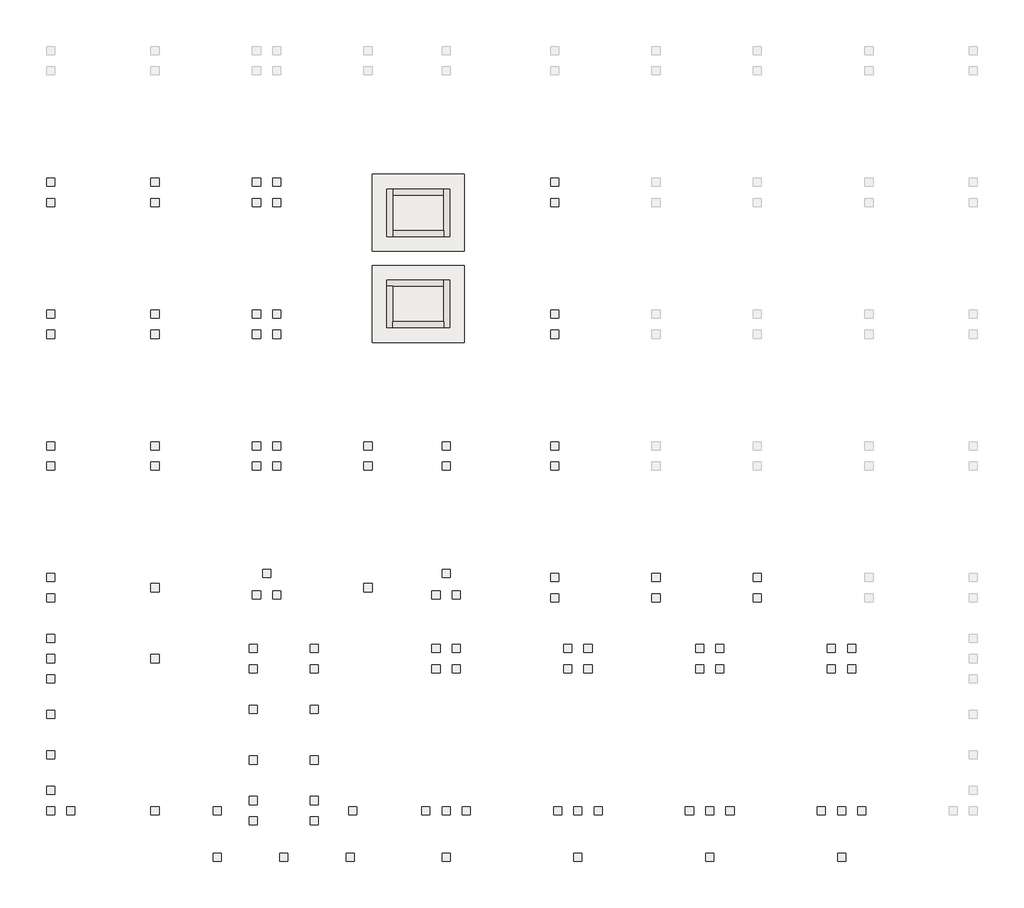
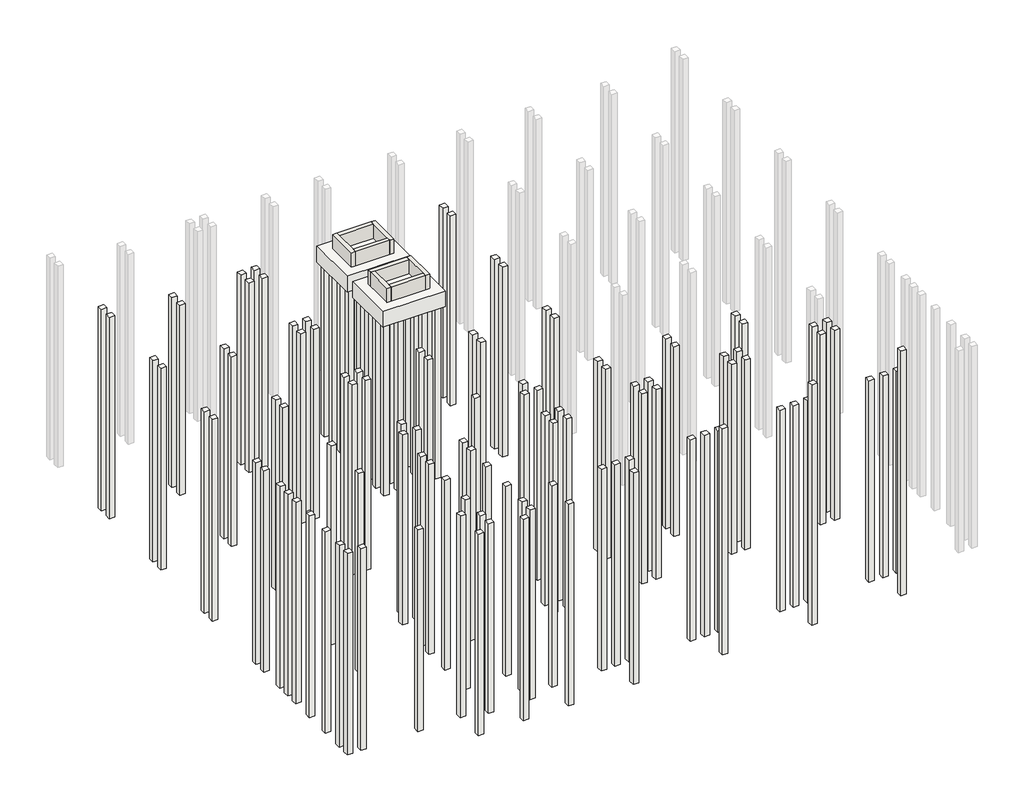
# Not in any storey, part 1 of 2: 143 footings, 8 walls.
# Revit data of these elements (continued)
# Element 100 (IfcFooting, "NLRS_17_SFO_TLB_funderingspaal geheid beton prefab-AV-MMBPC_gen_rsf : heipaal beton prefab_gen__bxh 400x400")
#   IfcGUID = "3loy75XKz2Rw4dS8JWiaqH"
#   Slanted Angle = 0.00°
#   NLRS_S_draagvermogen_trek = 0.00 kN
#   NLRS_S_draagvermogen_druk = 0.00 kN
#   Angle = 0.00°
#   IsExternal = yes
#   LoadBearing = yes
#   Slanted = 0
#   Phase Created = NLRS_nieuw
#   Materials on its faces: "NLRS_f2_beton prefab_gen_rsf"
# Element 101 (IfcFooting, "NLRS_17_SFO_TLB_funderingspaal geheid beton prefab-AV-MMBPC_gen_rsf : heipaal beton prefab_gen__bxh 400x400")
#   IfcGUID = "3loy75XKz2Rw4dS8JWiaqU"
#   Slanted Angle = 0.00°
#   NLRS_S_draagvermogen_trek = 0.00 kN
#   NLRS_S_draagvermogen_druk = 0.00 kN
#   Angle = 0.00°
#   IsExternal = yes
#   LoadBearing = yes
#   Slanted = 0
#   Phase Created = NLRS_nieuw
#   Materials on its faces: "NLRS_f2_beton prefab_gen_rsf"
# Element 102 (IfcFooting, "NLRS_17_SFO_TLB_funderingspaal geheid beton prefab-AV-MMBPC_gen_rsf : heipaal beton prefab_gen__bxh 400x400")
#   IfcGUID = "3loy75XKz2Rw4dS8JWiaqS"
#   Slanted Angle = 0.00°
#   NLRS_S_draagvermogen_trek = 0.00 kN
#   NLRS_S_draagvermogen_druk = 0.00 kN
#   Angle = 0.00°
#   IsExternal = yes
#   LoadBearing = yes
#   Slanted = 0
#   Phase Created = NLRS_nieuw
#   Materials on its faces: "NLRS_f2_beton prefab_gen_rsf"
# Element 103 (IfcFooting, "NLRS_17_SFO_TLB_funderingspaal geheid beton prefab-AV-MMBPC_gen_rsf : heipaal beton prefab_gen__bxh 400x400")
#   IfcGUID = "3loy75XKz2Rw4dS8JWiaq9"
#   Slanted Angle = 0.00°
#   NLRS_S_draagvermogen_trek = 0.00 kN
#   NLRS_S_draagvermogen_druk = 0.00 kN
#   Angle = 0.00°
#   IsExternal = yes
#   LoadBearing = yes
#   Slanted = 0
#   Phase Created = NLRS_nieuw
#   Materials on its faces: "NLRS_f2_beton prefab_gen_rsf"
# Element 104 (IfcFooting, "NLRS_17_SFO_TLB_funderingspaal geheid beton prefab-AV-MMBPC_gen_rsf : heipaal beton prefab_gen__bxh 400x400")
#   IfcGUID = "3loy75XKz2Rw4dS8JWiaqF"
#   Slanted Angle = 0.00°
#   NLRS_S_draagvermogen_trek = 0.00 kN
#   NLRS_S_draagvermogen_druk = 0.00 kN
#   Angle = 0.00°
#   IsExternal = yes
#   LoadBearing = yes
#   Slanted = 0
#   Phase Created = NLRS_nieuw
#   Materials on its faces: "NLRS_f2_beton prefab_gen_rsf"
# Element 105 (IfcFooting, "NLRS_17_SFO_TLB_funderingspaal geheid beton prefab-AV-MMBPC_gen_rsf : heipaal beton prefab_gen__bxh 400x400")
#   IfcGUID = "3loy75XKz2Rw4dS8JWia7f"
#   Slanted Angle = 0.00°
#   NLRS_S_draagvermogen_trek = 0.00 kN
#   NLRS_S_draagvermogen_druk = 0.00 kN
#   Angle = 0.00°
#   IsExternal = yes
#   LoadBearing = yes
#   Slanted = 0
#   Phase Created = NLRS_nieuw
#   Materials on its faces: "NLRS_f2_beton prefab_gen_rsf"
# Element 106 (IfcFooting, "NLRS_17_SFO_TLB_funderingspaal geheid beton prefab-AV-MMBPC_gen_rsf : heipaal beton prefab_gen__bxh 400x400")
#   IfcGUID = "3loy75XKz2Rw4dS8JWia6M"
#   Slanted Angle = 0.00°
#   NLRS_S_draagvermogen_trek = 0.00 kN
#   NLRS_S_draagvermogen_druk = 0.00 kN
#   Angle = 0.00°
#   IsExternal = yes
#   LoadBearing = yes
#   Slanted = 0
#   Phase Created = NLRS_nieuw
#   Materials on its faces: "NLRS_f2_beton prefab_gen_rsf"
# Element 107 (IfcFooting, "NLRS_17_SFO_TLB_funderingspaal geheid beton prefab-AV-MMBPC_gen_rsf : heipaal beton prefab_gen__bxh 400x400")
#   IfcGUID = "3loy75XKz2Rw4dS8JWiaPz"
#   Slanted Angle = 0.00°
#   NLRS_S_draagvermogen_trek = 0.00 kN
#   NLRS_S_draagvermogen_druk = 0.00 kN
#   Angle = 0.00°
#   IsExternal = yes
#   LoadBearing = yes
#   Slanted = 0
#   Phase Created = NLRS_nieuw
#   Materials on its faces: "NLRS_f2_beton prefab_gen_rsf"
# Element 108 (IfcFooting, "NLRS_17_SFO_TLB_funderingspaal geheid beton prefab-AV-MMBPC_gen_rsf : heipaal beton prefab_gen__bxh 400x400")
#   IfcGUID = "3yoae3mAzBRekDMiYpsxUC"
#   Slanted Angle = 0.00°
#   NLRS_S_draagvermogen_trek = 0.00 kN
#   NLRS_S_draagvermogen_druk = 0.00 kN
#   Angle = 0.00°
#   IsExternal = yes
#   LoadBearing = yes
#   Slanted = 0
#   Phase Created = NLRS_nieuw
#   Materials on its faces: "NLRS_f2_beton prefab_gen_rsf"
# Element 109 (IfcFooting, "NLRS_17_SFO_TLB_funderingspaal geheid beton prefab-AV-MMBPC_gen_rsf : heipaal beton prefab_gen__bxh 400x400")
#   IfcGUID = "3yoae3mAzBRekDMiYpsxUN"
#   Slanted Angle = 0.00°
#   NLRS_S_draagvermogen_trek = 0.00 kN
#   NLRS_S_draagvermogen_druk = 0.00 kN
#   Angle = 0.00°
#   IsExternal = yes
#   LoadBearing = yes
#   Slanted = 0
#   Phase Created = NLRS_nieuw
#   Materials on its faces: "NLRS_f2_beton prefab_gen_rsf"
# Element 110 (IfcFooting, "NLRS_17_SFO_TLB_funderingspaal geheid beton prefab-AV-MMBPC_gen_rsf : heipaal beton prefab_gen__bxh 400x400")
#   IfcGUID = "3yoae3mAzBRekDMiYpsxUU"
#   Slanted Angle = 0.00°
#   NLRS_S_draagvermogen_trek = 0.00 kN
#   NLRS_S_draagvermogen_druk = 0.00 kN
#   Angle = 0.00°
#   IsExternal = yes
#   LoadBearing = yes
#   Slanted = 0
#   Phase Created = NLRS_nieuw
#   Materials on its faces: "NLRS_f2_beton prefab_gen_rsf"
# Element 111 (IfcFooting, "NLRS_17_SFO_TLB_funderingspaal geheid beton prefab-AV-MMBPC_gen_rsf : heipaal beton prefab_gen__bxh 400x400")
#   IfcGUID = "3yoae3mAzBRekDMiYpsxVf"
#   Slanted Angle = 0.00°
#   NLRS_S_draagvermogen_trek = 0.00 kN
#   NLRS_S_draagvermogen_druk = 0.00 kN
#   Angle = 0.00°
#   IsExternal = yes
#   LoadBearing = yes
#   Slanted = 0
#   Phase Created = NLRS_nieuw
#   Materials on its faces: "NLRS_f2_beton prefab_gen_rsf"
# Element 112 (IfcFooting, "NLRS_17_SFO_TLB_funderingspaal geheid beton prefab-AV-MMBPC_gen_rsf : heipaal beton prefab_gen__bxh 400x400")
#   IfcGUID = "22y6L5gAz9AR8RjJaZzOrs"
#   Slanted Angle = 0.00°
#   NLRS_S_draagvermogen_trek = 0.00 kN
#   NLRS_S_draagvermogen_druk = 0.00 kN
#   Angle = 0.00°
#   IsExternal = yes
#   LoadBearing = yes
#   Slanted = 0
#   Phase Created = NLRS_nieuw
#   Materials on its faces: "NLRS_f2_beton prefab_gen_rsf"
# Element 113 (IfcFooting, "NLRS_17_SFO_TLB_funderingspaal geheid beton prefab-AV-MMBPC_gen_rsf : heipaal beton prefab_gen__bxh 400x400")
#   IfcGUID = "22y6L5gAz9AR8RjJaZzOqH"
#   Slanted Angle = 0.00°
#   NLRS_S_draagvermogen_trek = 0.00 kN
#   NLRS_S_draagvermogen_druk = 0.00 kN
#   Angle = 0.00°
#   IsExternal = yes
#   LoadBearing = yes
#   Slanted = 0
#   Phase Created = NLRS_nieuw
#   Materials on its faces: "NLRS_f2_beton prefab_gen_rsf"
# Element 114 (IfcFooting, "NLRS_17_SFO_TLB_funderingspaal geheid beton prefab-AV-MMBPC_gen_rsf : heipaal beton prefab_gen__bxh 400x400")
#   IfcGUID = "22y6L5gAz9AR8RjJaZzOo$"
#   Slanted Angle = 0.00°
#   NLRS_S_draagvermogen_trek = 0.00 kN
#   NLRS_S_draagvermogen_druk = 0.00 kN
#   Angle = 0.00°
#   IsExternal = yes
#   LoadBearing = yes
#   Slanted = 0
#   Phase Created = NLRS_nieuw
#   Materials on its faces: "NLRS_f2_beton prefab_gen_rsf"
# Element 115 (IfcFooting, "NLRS_17_SFO_TLB_funderingspaal geheid beton prefab-AV-MMBPC_gen_rsf : heipaal beton prefab_gen__bxh 400x400")
#   IfcGUID = "22y6L5gAz9AR8RjJaZzOn6"
#   Slanted Angle = 0.00°
#   NLRS_S_draagvermogen_trek = 0.00 kN
#   NLRS_S_draagvermogen_druk = 0.00 kN
#   Angle = 0.00°
#   IsExternal = yes
#   LoadBearing = yes
#   Slanted = 0
#   Phase Created = NLRS_nieuw
#   Materials on its faces: "NLRS_f2_beton prefab_gen_rsf"
# Element 116 (IfcFooting, "NLRS_17_SFO_TLB_funderingspaal geheid beton prefab-AV-MMBPC_gen_rsf : heipaal beton prefab_gen__bxh 400x400")
#   IfcGUID = "22y6L5gAz9AR8RjJaZzOmJ"
#   Slanted Angle = 0.00°
#   NLRS_S_draagvermogen_trek = 0.00 kN
#   NLRS_S_draagvermogen_druk = 0.00 kN
#   Angle = 0.00°
#   IsExternal = yes
#   LoadBearing = yes
#   Slanted = 0
#   Phase Created = NLRS_nieuw
#   Materials on its faces: "NLRS_f2_beton prefab_gen_rsf"
# Element 117 (IfcFooting, "NLRS_17_SFO_TLB_funderingspaal geheid beton prefab-AV-MMBPC_gen_rsf : heipaal beton prefab_gen__bxh 400x400")
#   IfcGUID = "22y6L5gAz9AR8RjJaZzOmD"
#   Slanted Angle = 0.00°
#   NLRS_S_draagvermogen_trek = 0.00 kN
#   NLRS_S_draagvermogen_druk = 0.00 kN
#   Angle = 0.00°
#   IsExternal = yes
#   LoadBearing = yes
#   Slanted = 0
#   Phase Created = NLRS_nieuw
#   Materials on its faces: "NLRS_f2_beton prefab_gen_rsf"
# Element 118 (IfcFooting, "NLRS_17_SFO_TLB_funderingspaal geheid beton prefab-AV-MMBPC_gen_rsf : heipaal beton prefab_gen__bxh 400x400")
#   IfcGUID = "22y6L5gAz9AR8RjJaZzOmk"
#   Slanted Angle = 0.00°
#   NLRS_S_draagvermogen_trek = 0.00 kN
#   NLRS_S_draagvermogen_druk = 0.00 kN
#   Angle = 0.00°
#   IsExternal = yes
#   LoadBearing = yes
#   Slanted = 0
#   Phase Created = NLRS_nieuw
#   Materials on its faces: "NLRS_f2_beton prefab_gen_rsf"
# Element 119 (IfcFooting, "NLRS_17_SFO_TLB_funderingspaal geheid beton prefab-AV-MMBPC_gen_rsf : heipaal beton prefab_gen__bxh 400x400")
#   IfcGUID = "22y6L5gAz9AR8RjJaZzOme"
#   Slanted Angle = 0.00°
#   NLRS_S_draagvermogen_trek = 0.00 kN
#   NLRS_S_draagvermogen_druk = 0.00 kN
#   Angle = 0.00°
#   IsExternal = yes
#   LoadBearing = yes
#   Slanted = 0
#   Phase Created = NLRS_nieuw
#   Materials on its faces: "NLRS_f2_beton prefab_gen_rsf"
# Element 120 (IfcFooting, "NLRS_17_SFO_TLB_funderingspaal geheid beton prefab-AV-MMBPC_gen_rsf : heipaal beton prefab_gen__bxh 400x400")
#   IfcGUID = "22y6L5gAz9AR8RjJaZzO$2"
#   Slanted Angle = 0.00°
#   NLRS_S_draagvermogen_trek = 0.00 kN
#   NLRS_S_draagvermogen_druk = 0.00 kN
#   Angle = 0.00°
#   IsExternal = yes
#   LoadBearing = yes
#   Slanted = 0
#   Phase Created = NLRS_nieuw
#   Materials on its faces: "NLRS_f2_beton prefab_gen_rsf"
# Element 121 (IfcFooting, "NLRS_17_SFO_TLB_funderingspaal geheid beton prefab-AV-MMBPC_gen_rsf : heipaal beton prefab_gen__bxh 400x400")
#   IfcGUID = "22y6L5gAz9AR8RjJaZzO$y"
#   Slanted Angle = 0.00°
#   NLRS_S_draagvermogen_trek = 0.00 kN
#   NLRS_S_draagvermogen_druk = 0.00 kN
#   Angle = 0.00°
#   IsExternal = yes
#   LoadBearing = yes
#   Slanted = 0
#   Phase Created = NLRS_nieuw
#   Materials on its faces: "NLRS_f2_beton prefab_gen_rsf"
# Element 122 (IfcFooting, "NLRS_17_SFO_TLB_funderingspaal geheid beton prefab-AV-MMBPC_gen_rsf : heipaal beton prefab_gen__bxh 400x400")
#   IfcGUID = "22y6L5gAz9AR8RjJaZzO$_"
#   Slanted Angle = 0.00°
#   NLRS_S_draagvermogen_trek = 0.00 kN
#   NLRS_S_draagvermogen_druk = 0.00 kN
#   Angle = 0.00°
#   IsExternal = yes
#   LoadBearing = yes
#   Slanted = 0
#   Phase Created = NLRS_nieuw
#   Materials on its faces: "NLRS_f2_beton prefab_gen_rsf"
# Element 123 (IfcFooting, "NLRS_17_SFO_TLB_funderingspaal geheid beton prefab-AV-MMBPC_gen_rsf : heipaal beton prefab_gen__bxh 400x400")
#   IfcGUID = "22y6L5gAz9AR8RjJaZzO$u"
#   Slanted Angle = 0.00°
#   NLRS_S_draagvermogen_trek = 0.00 kN
#   NLRS_S_draagvermogen_druk = 0.00 kN
#   Angle = 0.00°
#   IsExternal = yes
#   LoadBearing = yes
#   Slanted = 0
#   Phase Created = NLRS_nieuw
#   Materials on its faces: "NLRS_f2_beton prefab_gen_rsf"
# Element 124 (IfcFooting, "NLRS_17_SFO_TLB_funderingspaal geheid beton prefab-AV-MMBPC_gen_rsf : heipaal beton prefab_gen__bxh 400x400")
#   IfcGUID = "22y6L5gAz9AR8RjJaZzO$w"
#   Slanted Angle = 0.00°
#   NLRS_S_draagvermogen_trek = 0.00 kN
#   NLRS_S_draagvermogen_druk = 0.00 kN
#   Angle = 0.00°
#   IsExternal = yes
#   LoadBearing = yes
#   Slanted = 0
#   Phase Created = NLRS_nieuw
#   Materials on its faces: "NLRS_f2_beton prefab_gen_rsf"
# Element 125 (IfcFooting, "NLRS_17_SFO_TLB_funderingspaal geheid beton prefab-AV-MMBPC_gen_rsf : heipaal beton prefab_gen__bxh 400x400")
#   IfcGUID = "22y6L5gAz9AR8RjJaZzO$q"
#   Slanted Angle = 0.00°
#   NLRS_S_draagvermogen_trek = 0.00 kN
#   NLRS_S_draagvermogen_druk = 0.00 kN
#   Angle = 0.00°
#   IsExternal = yes
#   LoadBearing = yes
#   Slanted = 0
#   Phase Created = NLRS_nieuw
#   Materials on its faces: "NLRS_f2_beton prefab_gen_rsf"
# Element 126 (IfcFooting, "NLRS_17_SFO_TLB_funderingspaal geheid beton prefab-AV-MMBPC_gen_rsf : heipaal beton prefab_gen__bxh 400x400")
#   IfcGUID = "22y6L5gAz9AR8RjJaZzO$s"
#   Slanted Angle = 0.00°
#   NLRS_S_draagvermogen_trek = 0.00 kN
#   NLRS_S_draagvermogen_druk = 0.00 kN
#   Angle = 0.00°
#   IsExternal = yes
#   LoadBearing = yes
#   Slanted = 0
#   Phase Created = NLRS_nieuw
#   Materials on its faces: "NLRS_f2_beton prefab_gen_rsf"
# Element 127 (IfcFooting, "NLRS_17_SFO_TLB_funderingspaal geheid beton prefab-AV-MMBPC_gen_rsf : heipaal beton prefab_gen__bxh 400x400")
#   IfcGUID = "22y6L5gAz9AR8RjJaZzO$m"
#   Slanted Angle = 0.00°
#   NLRS_S_draagvermogen_trek = 0.00 kN
#   NLRS_S_draagvermogen_druk = 0.00 kN
#   Angle = 0.00°
#   IsExternal = yes
#   LoadBearing = yes
#   Slanted = 0
#   Phase Created = NLRS_nieuw
#   Materials on its faces: "NLRS_f2_beton prefab_gen_rsf"
# Element 128 (IfcFooting, "NLRS_17_SFO_TLB_funderingspaal geheid beton prefab-AV-MMBPC_gen_rsf : heipaal beton prefab_gen__bxh 400x400")
#   IfcGUID = "22y6L5gAz9AR8RjJaZzOuC"
#   Slanted Angle = 0.00°
#   NLRS_S_draagvermogen_trek = 0.00 kN
#   NLRS_S_draagvermogen_druk = 0.00 kN
#   Angle = 0.00°
#   IsExternal = yes
#   LoadBearing = yes
#   Slanted = 0
#   Phase Created = NLRS_nieuw
#   Materials on its faces: "NLRS_f2_beton prefab_gen_rsf"
# Element 129 (IfcFooting, "NLRS_17_SFO_TLB_funderingspaal geheid beton prefab-AV-MMBPC_gen_rsf : heipaal beton prefab_gen__bxh 400x400")
#   IfcGUID = "22y6L5gAz9AR8RjJaZzOuE"
#   Slanted Angle = 0.00°
#   NLRS_S_draagvermogen_trek = 0.00 kN
#   NLRS_S_draagvermogen_druk = 0.00 kN
#   Angle = 0.00°
#   IsExternal = yes
#   LoadBearing = yes
#   Slanted = 0
#   Phase Created = NLRS_nieuw
#   Materials on its faces: "NLRS_f2_beton prefab_gen_rsf"
# Element 130 (IfcFooting, "NLRS_17_SFO_TLB_funderingspaal geheid beton prefab-AV-MMBPC_gen_rsf : heipaal beton prefab_gen__bxh 400x400")
#   IfcGUID = "22y6L5gAz9AR8RjJaZzOu8"
#   Slanted Angle = 0.00°
#   NLRS_S_draagvermogen_trek = 0.00 kN
#   NLRS_S_draagvermogen_druk = 0.00 kN
#   Angle = 0.00°
#   IsExternal = yes
#   LoadBearing = yes
#   Slanted = 0
#   Phase Created = NLRS_nieuw
#   Materials on its faces: "NLRS_f2_beton prefab_gen_rsf"
# Element 131 (IfcFooting, "NLRS_17_SFO_TLB_funderingspaal geheid beton prefab-AV-MMBPC_gen_rsf : heipaal beton prefab_gen__bxh 400x400")
#   IfcGUID = "22y6L5gAz9AR8RjJaZzOuA"
#   Slanted Angle = 0.00°
#   NLRS_S_draagvermogen_trek = 0.00 kN
#   NLRS_S_draagvermogen_druk = 0.00 kN
#   Angle = 0.00°
#   IsExternal = yes
#   LoadBearing = yes
#   Slanted = 0
#   Phase Created = NLRS_nieuw
#   Materials on its faces: "NLRS_f2_beton prefab_gen_rsf"
# Element 132 (IfcFooting, "NLRS_17_SFO_TLB_funderingspaal geheid beton prefab-AV-MMBPC_gen_rsf : heipaal beton prefab_gen__bxh 400x400")
#   IfcGUID = "22y6L5gAz9AR8RjJaZzOu4"
#   Slanted Angle = 0.00°
#   NLRS_S_draagvermogen_trek = 0.00 kN
#   NLRS_S_draagvermogen_druk = 0.00 kN
#   Angle = 0.00°
#   IsExternal = yes
#   LoadBearing = yes
#   Slanted = 0
#   Phase Created = NLRS_nieuw
#   Materials on its faces: "NLRS_f2_beton prefab_gen_rsf"
# Element 133 (IfcFooting, "NLRS_17_SFO_TLB_funderingspaal geheid beton prefab-AV-MMBPC_gen_rsf : heipaal beton prefab_gen__bxh 400x400")
#   IfcGUID = "22y6L5gAz9AR8RjJaZzOu6"
#   Slanted Angle = 0.00°
#   NLRS_S_draagvermogen_trek = 0.00 kN
#   NLRS_S_draagvermogen_druk = 0.00 kN
#   Angle = 0.00°
#   IsExternal = yes
#   LoadBearing = yes
#   Slanted = 0
#   Phase Created = NLRS_nieuw
#   Materials on its faces: "NLRS_f2_beton prefab_gen_rsf"
# Element 134 (IfcFooting, "NLRS_17_SFO_TLB_funderingspaal geheid beton prefab-AV-MMBPC_gen_rsf : heipaal beton prefab_gen__bxh 400x400")
#   IfcGUID = "22y6L5gAz9AR8RjJaZzOu0"
#   Slanted Angle = 0.00°
#   NLRS_S_draagvermogen_trek = 0.00 kN
#   NLRS_S_draagvermogen_druk = 0.00 kN
#   Angle = 0.00°
#   IsExternal = yes
#   LoadBearing = yes
#   Slanted = 0
#   Phase Created = NLRS_nieuw
#   Materials on its faces: "NLRS_f2_beton prefab_gen_rsf"
# Element 135 (IfcFooting, "NLRS_17_SFO_TLB_funderingspaal geheid beton prefab-AV-MMBPC_gen_rsf : heipaal beton prefab_gen__bxh 400x400")
#   IfcGUID = "22y6L5gAz9AR8RjJaZzOu2"
#   Slanted Angle = 0.00°
#   NLRS_S_draagvermogen_trek = 0.00 kN
#   NLRS_S_draagvermogen_druk = 0.00 kN
#   Angle = 0.00°
#   IsExternal = yes
#   LoadBearing = yes
#   Slanted = 0
#   Phase Created = NLRS_nieuw
#   Materials on its faces: "NLRS_f2_beton prefab_gen_rsf"
# Element 136 (IfcFooting, "NLRS_17_SFO_TLB_funderingspaal geheid beton prefab-AV-MMBPC_gen_rsf : heipaal beton prefab_gen__bxh 400x400")
#   IfcGUID = "22y6L5gAz9AR8RjJaZzOuy"
#   Slanted Angle = 0.00°
#   NLRS_S_draagvermogen_trek = 0.00 kN
#   NLRS_S_draagvermogen_druk = 0.00 kN
#   Angle = 0.00°
#   IsExternal = yes
#   LoadBearing = yes
#   Slanted = 0
#   Phase Created = NLRS_nieuw
#   Materials on its faces: "NLRS_f2_beton prefab_gen_rsf"
# Element 137 (IfcFooting, "NLRS_17_SFO_TLB_funderingspaal geheid beton prefab-AV-MMBPC_gen_rsf : heipaal beton prefab_gen__bxh 400x400")
#   IfcGUID = "22y6L5gAz9AR8RjJaZzOu_"
#   Slanted Angle = 0.00°
#   NLRS_S_draagvermogen_trek = 0.00 kN
#   NLRS_S_draagvermogen_druk = 0.00 kN
#   Angle = 0.00°
#   IsExternal = yes
#   LoadBearing = yes
#   Slanted = 0
#   Phase Created = NLRS_nieuw
#   Materials on its faces: "NLRS_f2_beton prefab_gen_rsf"
# Element 138 (IfcFooting, "NLRS_17_SFO_TLB_funderingspaal geheid beton prefab-AV-MMBPC_gen_rsf : heipaal beton prefab_gen__bxh 400x400")
#   IfcGUID = "22y6L5gAz9AR8RjJaZzOuu"
#   Slanted Angle = 0.00°
#   NLRS_S_draagvermogen_trek = 0.00 kN
#   NLRS_S_draagvermogen_druk = 0.00 kN
#   Angle = 0.00°
#   IsExternal = yes
#   LoadBearing = yes
#   Slanted = 0
#   Phase Created = NLRS_nieuw
#   Materials on its faces: "NLRS_f2_beton prefab_gen_rsf"
# Element 139 (IfcFooting, "NLRS_17_SFO_TLB_funderingspaal geheid beton prefab-AV-MMBPC_gen_rsf : heipaal beton prefab_gen__bxh 400x400")
#   IfcGUID = "22y6L5gAz9AR8RjJaZzOuw"
#   Slanted Angle = 0.00°
#   NLRS_S_draagvermogen_trek = 0.00 kN
#   NLRS_S_draagvermogen_druk = 0.00 kN
#   Angle = 0.00°
#   IsExternal = yes
#   LoadBearing = yes
#   Slanted = 0
#   Phase Created = NLRS_nieuw
#   Materials on its faces: "NLRS_f2_beton prefab_gen_rsf"
# Element 140 (IfcFooting, "NLRS_17_SFO_TLB_funderingspaal geheid beton prefab-AV-MMBPC_gen_rsf : heipaal beton prefab_gen__bxh 400x400")
#   IfcGUID = "22y6L5gAz9AR8RjJaZzOuq"
#   Slanted Angle = 0.00°
#   NLRS_S_draagvermogen_trek = 0.00 kN
#   NLRS_S_draagvermogen_druk = 0.00 kN
#   Angle = 0.00°
#   IsExternal = yes
#   LoadBearing = yes
#   Slanted = 0
#   Phase Created = NLRS_nieuw
#   Materials on its faces: "NLRS_f2_beton prefab_gen_rsf"
# Element 141 (IfcFooting, "NLRS_17_SFO_TLB_funderingspaal geheid beton prefab-AV-MMBPC_gen_rsf : heipaal beton prefab_gen__bxh 400x400")
#   IfcGUID = "22y6L5gAz9AR8RjJaZzOus"
#   Slanted Angle = 0.00°
#   NLRS_S_draagvermogen_trek = 0.00 kN
#   NLRS_S_draagvermogen_druk = 0.00 kN
#   Angle = 0.00°
#   IsExternal = yes
#   LoadBearing = yes
#   Slanted = 0
#   Phase Created = NLRS_nieuw
#   Materials on its faces: "NLRS_f2_beton prefab_gen_rsf"
# Element 142 (IfcFooting, "NLRS_17_SFO_TLB_funderingspaal geheid beton prefab-AV-MMBPC_gen_rsf : heipaal beton prefab_gen__bxh 400x400")
#   IfcGUID = "22y6L5gAz9AR8RjJaZzOum"
#   Slanted Angle = 0.00°
#   NLRS_S_draagvermogen_trek = 0.00 kN
#   NLRS_S_draagvermogen_druk = 0.00 kN
#   Angle = 0.00°
#   IsExternal = yes
#   LoadBearing = yes
#   Slanted = 0
#   Phase Created = NLRS_nieuw
#   Materials on its faces: "NLRS_f2_beton prefab_gen_rsf"
# Element 143 (IfcFooting, "NLRS_17_SFO_TLB_funderingspaal geheid beton prefab-AV-MMBPC_gen_rsf : heipaal beton prefab_gen__bxh 400x400")
#   IfcGUID = "22y6L5gAz9AR8RjJaZzOuo"
#   Slanted Angle = 0.00°
#   NLRS_S_draagvermogen_trek = 0.00 kN
#   NLRS_S_draagvermogen_druk = 0.00 kN
#   Angle = 0.00°
#   IsExternal = yes
#   LoadBearing = yes
#   Slanted = 0
#   Phase Created = NLRS_nieuw
#   Materials on its faces: "NLRS_f2_beton prefab_gen_rsf"
# Element 144 (IfcWall, "NLRS_16_WA_beton ihw 300_gen_rsf")
#   IfcGUID = "22y6L5gAz9AR8RjJaZzOY4"
#   Comments = ""
#   Top Offset = 0 mm
#   Base Offset = 0 mm
#   wall height = 1100 mm
#   IsExternal = yes
#   LoadBearing = yes
#   Phase Created = NLRS_nieuw
#   Base Constraint = -02_bk ruwe vloer liftput
#   Top Constraint = -01_ok ruwe vloer
#   Materials on its faces: "NLRS_f2_beton ihwg_gen_rsf"
# Element 145 (IfcWall, "NLRS_16_WA_beton ihw 300_gen_rsf")
#   IfcGUID = "22y6L5gAz9AR8RjJaZzOY6"
#   Comments = ""
#   Top Offset = 0 mm
#   Base Offset = 0 mm
#   wall height = 1100 mm
#   IsExternal = yes
#   LoadBearing = yes
#   Phase Created = NLRS_nieuw
#   Base Constraint = -02_bk ruwe vloer liftput
#   Top Constraint = -01_ok ruwe vloer
#   Materials on its faces: "NLRS_f2_beton ihwg_gen_rsf"
# Element 146 (IfcWall, "NLRS_16_WA_beton ihw 300_gen_rsf")
#   IfcGUID = "22y6L5gAz9AR8RjJaZzOY0"
#   Comments = ""
#   Top Offset = 0 mm
#   Base Offset = 0 mm
#   wall height = 1100 mm
#   IsExternal = yes
#   LoadBearing = yes
#   Phase Created = NLRS_nieuw
#   Base Constraint = -02_bk ruwe vloer liftput
#   Top Constraint = -01_ok ruwe vloer
#   Materials on its faces: "NLRS_f2_beton ihwg_gen_rsf"
# Element 147 (IfcWall, "NLRS_16_WA_beton ihw 300_gen_rsf")
#   IfcGUID = "22y6L5gAz9AR8RjJaZzOY2"
#   Comments = ""
#   Top Offset = 0 mm
#   Base Offset = 0 mm
#   wall height = 1100 mm
#   IsExternal = yes
#   LoadBearing = yes
#   Phase Created = NLRS_nieuw
#   Base Constraint = -02_bk ruwe vloer liftput
#   Top Constraint = -01_ok ruwe vloer
#   Materials on its faces: "NLRS_f2_beton ihwg_gen_rsf"
# Element 148 (IfcWall, "NLRS_16_WA_beton ihw 300_gen_rsf")
#   IfcGUID = "22y6L5gAz9AR8RjJaZzOYy"
#   Comments = ""
#   Top Offset = 0 mm
#   Base Offset = 0 mm
#   wall height = 1100 mm
#   IsExternal = yes
#   LoadBearing = yes
#   Phase Created = NLRS_nieuw
#   Base Constraint = -02_bk ruwe vloer liftput
#   Top Constraint = -01_ok ruwe vloer
#   Materials on its faces: "NLRS_f2_beton ihwg_gen_rsf"
# Element 149 (IfcWall, "NLRS_16_WA_beton ihw 300_gen_rsf")
#   IfcGUID = "22y6L5gAz9AR8RjJaZzOY_"
#   Comments = ""
#   Top Offset = 0 mm
#   Base Offset = 0 mm
#   wall height = 1100 mm
#   IsExternal = yes
#   LoadBearing = yes
#   Phase Created = NLRS_nieuw
#   Base Constraint = -02_bk ruwe vloer liftput
#   Top Constraint = -01_ok ruwe vloer
#   Materials on its faces: "NLRS_f2_beton ihwg_gen_rsf"
# Element 150 (IfcWall, "NLRS_16_WA_beton ihw 300_gen_rsf")
#   IfcGUID = "22y6L5gAz9AR8RjJaZzOYu"
#   Comments = ""
#   Top Offset = 0 mm
#   Base Offset = 0 mm
#   wall height = 1100 mm
#   IsExternal = yes
#   LoadBearing = yes
#   Phase Created = NLRS_nieuw
#   Base Constraint = -02_bk ruwe vloer liftput
#   Top Constraint = -01_ok ruwe vloer
#   Materials on its faces: "NLRS_f2_beton ihwg_gen_rsf"
# Element 151 (IfcWall, "NLRS_16_WA_beton ihw 300_gen_rsf")
#   IfcGUID = "22y6L5gAz9AR8RjJaZzOYw"
#   Comments = ""
#   Top Offset = 0 mm
#   Base Offset = 0 mm
#   wall height = 1100 mm
#   IsExternal = yes
#   LoadBearing = yes
#   Phase Created = NLRS_nieuw
#   Base Constraint = -02_bk ruwe vloer liftput
#   Top Constraint = -01_ok ruwe vloer
#   Materials on its faces: "NLRS_f2_beton ihwg_gen_rsf"
# Materials
#   "NLRS_f2_beton ihwg_gen_rsf": class "F - Niet gebakken kunststeen", colour RGB 129 133 118, transparency 0, Keynote = "f2", Manufacturer = "Revit Standards Foundation", URL = "www.revitstandards.org", Description = "beton ihwg", Cost = 0
#   "NLRS_f2_beton prefab_gen_rsf": class "F - Niet gebakken kunststeen", colour RGB 129 133 118, transparency 0, Keynote = "f2", Manufacturer = "Revit Standards Foundation", URL = "www.revitstandards.org", Description = "beton prefab", Cost = 0
